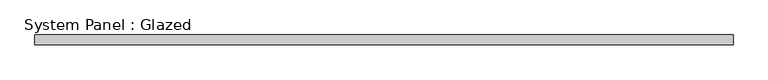
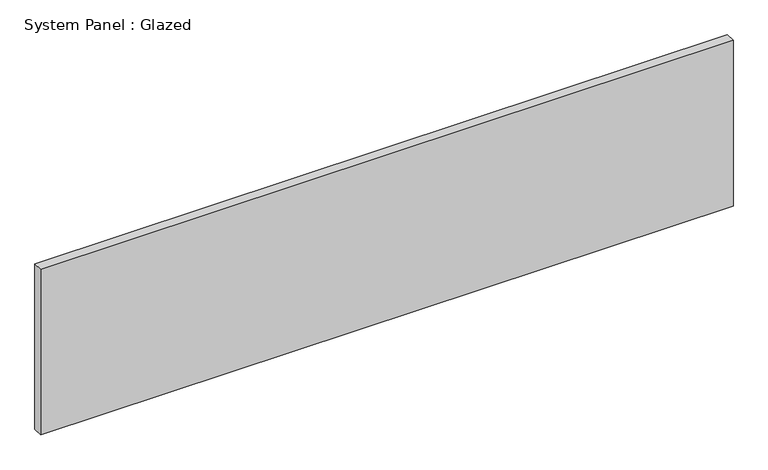
"""IFC4 building model written with IfcOpenShell, lengths in millimetres: plate geometry, System Panel : Glazed."""

from ifc_helpers import new_model, si_unit, origin, origin_with_axes, place, context, project, spatial, polyline, outline, extrude, source, transform, mapped, element, save


def system_panel_glazed_87c86ac8(model_context):
    return source(origin(), model_context, "Body", "SweptSolid", [
        extrude(outline(polyline([(890.0, 24.5), (-890.0, 24.5), (-890.0, 49.5), (890.0, 49.5), (890.0, 24.5)])), origin_with_axes(), (0.0, 0.0, 1.0), 450.0),
    ])


if __name__ == "__main__":
    model = new_model("IFC4")
    model_context = context("Model", 3, world=origin())
    ifc_project = project(units=[si_unit("LENGTHUNIT", "METRE", prefix="MILLI")], contexts=[model_context])
    site = spatial("IfcSite", under=ifc_project)
    building = spatial("IfcBuilding", under=site)
    placement = place(None, origin())
    system_panel_glazed_shape = system_panel_glazed_87c86ac8(model_context)
    element("IfcPlate", 1, ObjectType="System Panel : Glazed", at=placement, inside=building, context=model_context, shape_type="MappedRepresentation", body=[
        mapped(system_panel_glazed_shape, transform((0.0, 0.0, 0.0), x_axis=(1.0, 0.0, 0.0), y_axis=(0.0, 1.0, 0.0), z_axis=(0.0, 0.0, 1.0))),
    ])
    save(model, "model.ifc")

# Revit data of these elements
# Type "System Panel : Glazed"
#   Keynote = "H11"
#   Construction Type Id = "GSP4R"
#   Analytic Construction = "1/8 in Pilkington single glazing"
#   Visual Light Transmittance = 0.9
#   Solar Heat Gain Coefficient = 0.86
#   Heat Transfer Coefficient (U) = 6.7069 W/(m²·K)
# Element 1 (IfcPlate, "System Panel : Glazed")
#   Materials on its faces: "Glass"
# Materials
#   "Glass": class "Glass", colour RGB 0 128 192, transparency 0.9, Description = "Soda Lime Glass", Cost = 0
